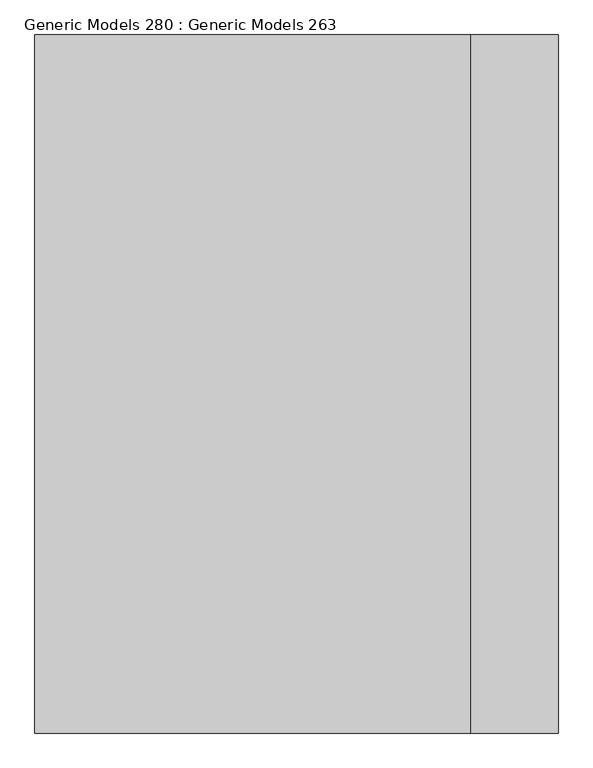
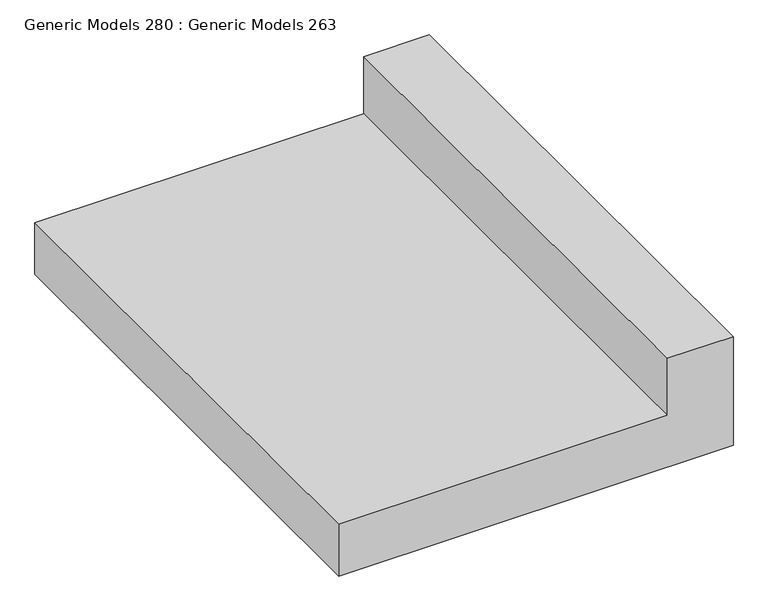
"""IFC4 building model written with IfcOpenShell, lengths in millimetres: proxy geometry, Generic Models 280 : Generic Models 263."""

from ifc_helpers import new_model, si_unit, frame, origin, place, context, project, spatial, polyline, outline, extrude, source, transform, mapped, element, save


def generic_models_280_generic_models_263_4ff5fa89(model_context):
    return source(origin(), model_context, "Body", "SweptSolid", [
        extrude(outline(polyline([(-381.0, 62776.3797726), (-381.0, 62014.3797726), (-508.0, 62014.3797726), (-508.0, 62928.7797726), (-241.3, 62928.7797726), (-241.3, 62776.3797726), (-381.0, 62776.3797726)])), frame((0.0, -94.4486541, 0.0), z_axis=(0.0, 1.0, 0.0), x_axis=(0.0, 0.0, 1.0)), (0.0, 0.0, 1.0), 1219.2),
    ])


if __name__ == "__main__":
    model = new_model("IFC4")
    model_context = context("Model", 3, world=origin())
    ifc_project = project(units=[si_unit("LENGTHUNIT", "METRE", prefix="MILLI")], contexts=[model_context])
    site = spatial("IfcSite", under=ifc_project)
    building = spatial("IfcBuilding", under=site)
    placement = place(None, origin())
    generic_models_280_generic_models_263_shape = generic_models_280_generic_models_263_4ff5fa89(model_context)
    element("IfcBuildingElementProxy", 1, Name="Generic Models 280 : Generic Models 263", ObjectType="Generic Models 280 : Generic Models 263", at=placement, inside=building, context=model_context, shape_type="MappedRepresentation", body=[
        mapped(generic_models_280_generic_models_263_shape, transform((0.0, 0.0, 0.0), x_axis=(1.0, 0.0, 0.0), y_axis=(0.0, 1.0, 0.0), z_axis=(0.0, 0.0, 1.0))),
    ])
    save(model, "model.ifc")

# Revit data of these elements
# Element 1 (IfcBuildingElementProxy, "Generic Models 280 : Generic Models 263")
#   Materials on its faces: "5\" MIN. COMPACTED BASE AGGREGATE UNDER CURB"
# Materials
#   "5\" MIN. COMPACTED BASE AGGREGATE UNDER CURB": class "Miscellaneous", colour RGB 183 184 198, transparency 0, Cost = 0
